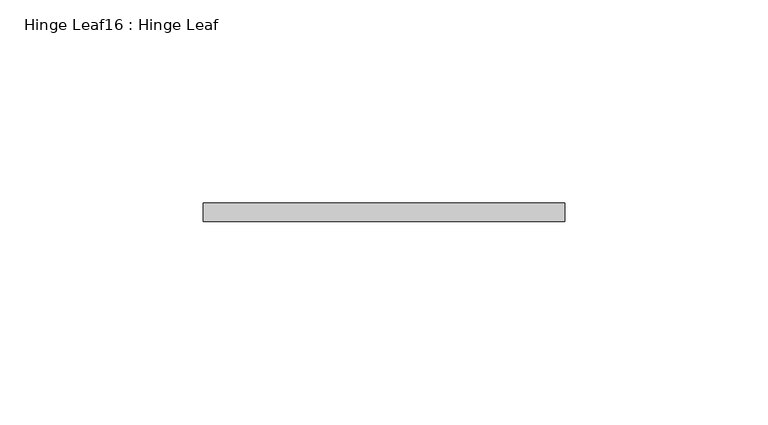
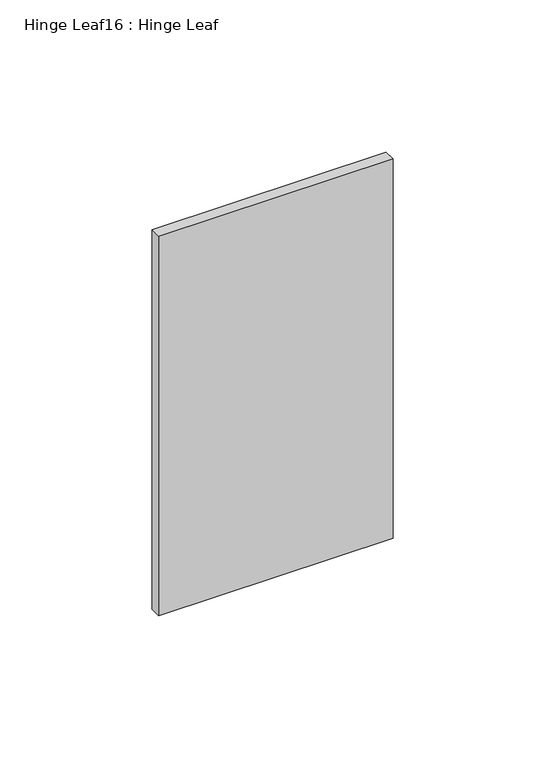
"""IFC4 building model written with IfcOpenShell, lengths in millimetres: proxy geometry, Hinge Leaf16 : Hinge Leaf."""

from ifc_helpers import new_model, si_unit, frame, origin, place, context, project, spatial, polyline, outline, extrude, source, transform, mapped, element, save


def hinge_leaf16_hinge_leaf_89afeb32(model_context):
    return source(origin(), model_context, "Body", "SweptSolid", [
        extrude(outline(polyline([(587327.7934739, -534104.7943841), (587416.6934739, -534104.7943841), (587416.6934739, -534109.3663841), (587327.7934739, -534109.3663841), (587327.7934739, -534104.7943841)])), frame((0.0, 0.0, 1936.75), z_axis=(0.0, 0.0, 1.0), x_axis=(1.0, 0.0, 0.0)), (0.0, 0.0, 1.0), 152.4),
    ])


if __name__ == "__main__":
    model = new_model("IFC4")
    model_context = context("Model", 3, world=origin())
    ifc_project = project(units=[si_unit("LENGTHUNIT", "METRE", prefix="MILLI")], contexts=[model_context])
    site = spatial("IfcSite", under=ifc_project)
    building = spatial("IfcBuilding", under=site)
    placement = place(None, origin())
    hinge_leaf16_hinge_leaf_shape = hinge_leaf16_hinge_leaf_89afeb32(model_context)
    element("IfcBuildingElementProxy", 1, Name="Hinge Leaf16 : Hinge Leaf", ObjectType="Hinge Leaf16 : Hinge Leaf", at=placement, inside=building, context=model_context, shape_type="MappedRepresentation", body=[
        mapped(hinge_leaf16_hinge_leaf_shape, transform((0.0, 0.0, 0.0), x_axis=(1.0, 0.0, 0.0), y_axis=(0.0, 1.0, 0.0), z_axis=(0.0, 0.0, 1.0))),
    ])
    save(model, "model.ifc")

# Revit data of these elements
# Element 1 (IfcBuildingElementProxy, "Hinge Leaf16 : Hinge Leaf")
#   Materials on its faces: "6\"X6\" WELD-ON STL BUTT HINGE"
# Materials
#   "6\"X6\" WELD-ON STL BUTT HINGE": class "Metal", colour RGB 189 187 185, transparency 0, Description = "Carbon steel", Cost = 0
